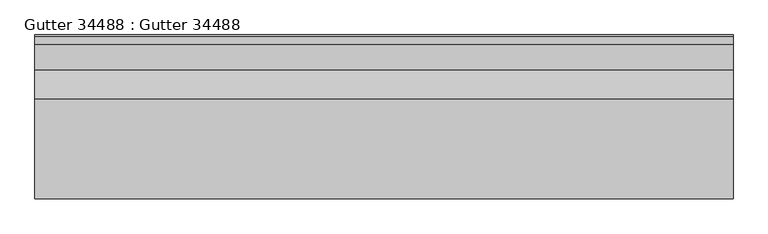
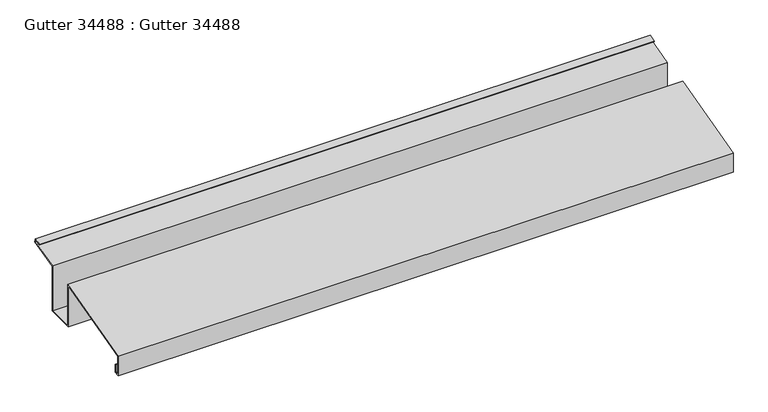
"""IFC4 building model written with IfcOpenShell, lengths in millimetres: proxy geometry, Gutter 34488 : Gutter 34488."""

from ifc_helpers import new_model, si_unit, frame, origin, place, context, project, spatial, polyline, outline, extrude, source, transform, mapped, element, save


def gutter_34488_gutter_34488_4af62660(model_context):
    return source(origin(), model_context, "Body", "SweptSolid", [
        extrude(outline(polyline([(-5603.5887201, 42700.9879789), (-5603.5887201, 42673.0479789), (-5621.3687201, 42673.0479789), (-5621.3687201, 42739.4471419), (-5336.549844, 42814.8665333), (-5336.549844, 42672.141563), (-5251.515638, 42672.141563), (-5251.515638, 42825.9077053), (-5154.761123, 42850.915099), (-5156.7473957, 42858.6000602), (-5177.4967906, 42853.237124), (-5178.0926724, 42855.5426123), (-5155.0377891, 42861.5014303), (-5151.8597529, 42849.2054925), (-5249.134388, 42824.0636673), (-5249.134388, 42669.601563), (-5339.089844, 42669.601563), (-5339.089844, 42811.566406), (-5618.8287201, 42737.492187), (-5618.8287201, 42675.5879789), (-5606.1287201, 42675.5879789), (-5606.1287201, 42700.9879789), (-5603.5887201, 42700.9879789)])), frame((12382.7678845, 0.0, 0.0), z_axis=(1.0, 0.0, 0.0), x_axis=(0.0, 1.0, 0.0)), (0.0, 0.0, 1.0), 2000.25),
    ])


if __name__ == "__main__":
    model = new_model("IFC4")
    model_context = context("Model", 3, world=origin())
    ifc_project = project(units=[si_unit("LENGTHUNIT", "METRE", prefix="MILLI")], contexts=[model_context])
    site = spatial("IfcSite", under=ifc_project)
    building = spatial("IfcBuilding", under=site)
    placement = place(None, origin())
    gutter_34488_gutter_34488_shape = gutter_34488_gutter_34488_4af62660(model_context)
    element("IfcBuildingElementProxy", 1, Name="Gutter 34488 : Gutter 34488", ObjectType="Gutter 34488 : Gutter 34488", at=placement, inside=building, context=model_context, shape_type="MappedRepresentation", body=[
        mapped(gutter_34488_gutter_34488_shape, transform((0.0, 0.0, 0.0), x_axis=(1.0, 0.0, 0.0), y_axis=(0.0, 1.0, 0.0), z_axis=(0.0, 0.0, 1.0))),
    ])
    save(model, "model.ifc")

# Revit data of these elements
# Type "Gutter 34488 : Gutter 34488"
#   NameOverride = "Gutter"
# Element 1 (IfcBuildingElementProxy, "Gutter 34488 : Gutter 34488")
#   Materials on its faces: "CONT. SEAMLESS 16 GA COPPER BRAKE METAL GUTTER"
# Materials
#   "CONT. SEAMLESS 16 GA COPPER BRAKE METAL GUTTER": class "Unassigned", colour RGB 128 128 128, transparency 0
